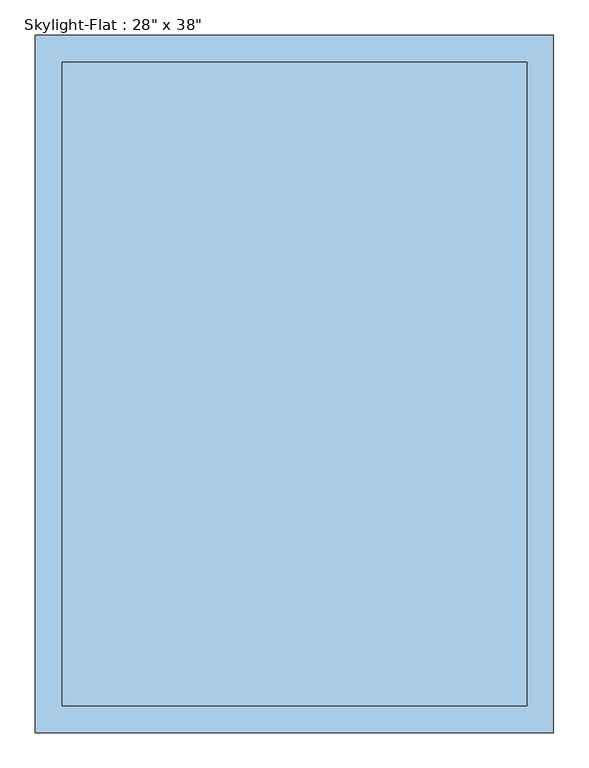
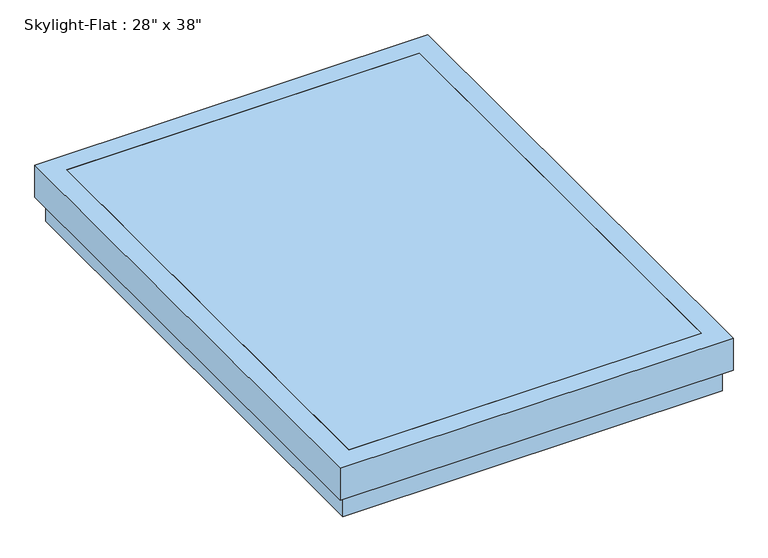
"""IFC4 building model written with IfcOpenShell, lengths in millimetres: window geometry."""

from ifc_helpers import new_model, si_unit, frame, origin, place, context, project, spatial, polyline, outline, extrude, faceted_brep, source, transform, mapped, element, save


def window_ea9d9d01(model_context):
    return source(origin(), model_context, "Body", "SolidModel", [
        extrude(outline(polyline([(330.2, 457.2), (330.2, -457.2), (-330.2, -457.2), (-330.2, 457.2), (330.2, 457.2)])), frame((0.0, 0.0, 4080.03375), z_axis=(0.0, 0.0, 1.0), x_axis=(1.0, 0.0, 0.0)), (0.0, 0.0, 1.0), 5.55625),
        faceted_brep([(368.3, 495.3, 4022.09), (368.3, 495.3, 4085.59), (368.3, -495.3, 4085.59), (368.3, -495.3, 4022.09), (355.6, 482.6, 4060.19), (355.6, 482.6, 4022.09), (355.6, -482.6, 4022.09), (355.6, -482.6, 4060.19), (330.2, 457.2, 4085.59), (330.2, 457.2, 4060.19), (330.2, -457.2, 4060.19), (330.2, -457.2, 4085.59), (-368.3, -495.3, 4085.59), (-368.3, -495.3, 4022.09), (-355.6, -482.6, 4022.09), (-355.6, -482.6, 4060.19), (-330.2, -457.2, 4060.19), (-330.2, -457.2, 4085.59), (-368.3, 495.3, 4085.59), (-368.3, 495.3, 4022.09), (-355.6, 482.6, 4022.09), (-355.6, 482.6, 4060.19), (-330.2, 457.2, 4060.19), (-330.2, 457.2, 4085.59)], [[[0, 1, 2, 3]], [[4, 5, 6, 7]], [[8, 9, 10, 11]], [[3, 2, 12, 13]], [[7, 6, 14, 15]], [[11, 10, 16, 17]], [[13, 12, 18, 19]], [[15, 14, 20, 21]], [[17, 16, 22, 23]], [[1, 18, 12, 2], [11, 17, 23, 8]], [[19, 18, 1, 0]], [[3, 13, 19, 0], [5, 20, 14, 6]], [[21, 20, 5, 4]], [[7, 15, 21, 4], [9, 22, 16, 10]], [[23, 22, 9, 8]]]),
        faceted_brep([(355.6, 482.6, 3977.64), (355.6, 482.6, 4060.19), (355.6, -482.6, 4060.19), (355.6, -482.6, 3977.64), (292.1, 419.1, 4034.79), (292.1, 419.1, 3977.64), (292.1, -419.1, 3977.64), (292.1, -419.1, 4034.79), (330.2, 457.2, 4060.19), (330.2, 457.2, 4034.79), (330.2, -457.2, 4034.79), (330.2, -457.2, 4060.19), (-355.6, -482.6, 4060.19), (-355.6, -482.6, 3977.64), (-292.1, -419.1, 3977.64), (-292.1, -419.1, 4034.79), (-330.2, -457.2, 4034.79), (-330.2, -457.2, 4060.19), (-355.6, 482.6, 4060.19), (-355.6, 482.6, 3977.64), (-292.1, 419.1, 3977.64), (-292.1, 419.1, 4034.79), (-330.2, 457.2, 4034.79), (-330.2, 457.2, 4060.19)], [[[0, 1, 2, 3]], [[4, 5, 6, 7]], [[8, 9, 10, 11]], [[3, 2, 12, 13]], [[7, 6, 14, 15]], [[11, 10, 16, 17]], [[13, 12, 18, 19]], [[15, 14, 20, 21]], [[17, 16, 22, 23]], [[19, 18, 1, 0]], [[3, 13, 19, 0], [5, 20, 14, 6]], [[21, 20, 5, 4]], [[9, 22, 16, 10], [7, 15, 21, 4]], [[23, 22, 9, 8]], [[1, 18, 12, 2], [11, 17, 23, 8]]]),
    ])


if __name__ == "__main__":
    model = new_model("IFC4")
    model_context = context("Model", 3, world=origin())
    ifc_project = project(units=[si_unit("LENGTHUNIT", "METRE", prefix="MILLI")], contexts=[model_context])
    site = spatial("IfcSite", under=ifc_project)
    building = spatial("IfcBuilding", under=site)
    placement = place(None, origin())
    window_shape = window_ea9d9d01(model_context)
    element("IfcWindow", 1, ObjectType="Skylight-Flat : 28\" x 38\"", at=placement, inside=building, context=model_context, shape_type="MappedRepresentation", body=[
        mapped(window_shape, transform((0.0, 0.0, 0.0), x_axis=(1.0, 0.0, 0.0), y_axis=(0.0, 1.0, 0.0), z_axis=(0.0, 0.0, 1.0))),
    ])
    save(model, "model.ifc")

# Revit data of these elements
# Type "Skylight-Flat : 28\" x 38\""
#   Type Mark = "10"
#   Fire Rating = "0.5h"
#   Assembly Code = "B3020110"
#   Analytic Construction = "1/8 in Pilkington single glazing"
#   Visual Light Transmittance = 0.9
#   Thermal Resistance (R) = 0.9899 (h·ft²·°F)/BTU
#   Solar Heat Gain Coefficient = 0.78
#   Rough Width = 2.375 ft
#   Rough Height = 3.208333 ft
#   Heat Transfer Coefficient (U) = 0.6496 BTU/(h·ft²·°F)
#   Base Height = 0.270833 ft
#   Height = 3.166667 ft
#   Width = 2.333333 ft
#   Glass Panel Material = Glass
#   Frame Material = Metal - Bronze, Light Brush
# Element 1 (IfcWindow, "Skylight-Flat : 28\" x 38\"")
#   Materials on its faces: "Metal - Bronze, Light Brush", "Glass"
# Materials
#   "Glass": class "Glass", colour RGB 0 128 192, transparency 0.75, Description = "Soda Lime Glass", Cost = 0
#   "Metal - Bronze, Light Brush": class "Metal", colour RGB 113 80 70, transparency 0
